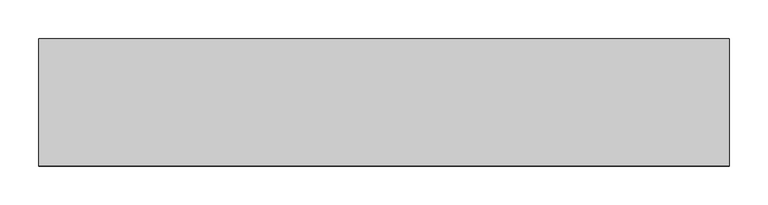
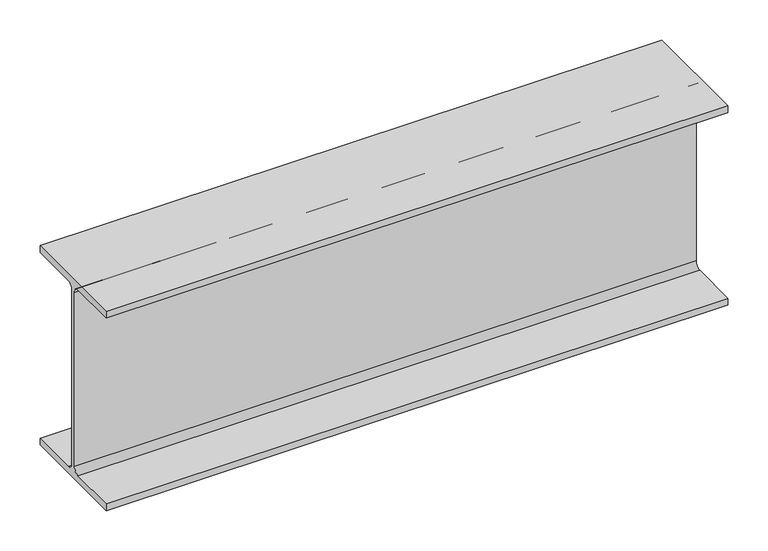
"""IFC4 building model written with IfcOpenShell, lengths in millimetres: beam geometry, Steel Beam_H-KSD3502 : H_SB_ASB_H-300x150x6.5x9."""

from ifc_helpers import new_model, si_unit, point, frame, frame_2d, origin, place, context, project, spatial, polyline, circle_curve, trimmed, segment, composite_curve, outline, extrude, source, transform, mapped, element, save


def beam_bd3552e1(model_context):
    return source(origin(), model_context, "Body", "SweptSolid", [
        extrude(outline(composite_curve([segment(polyline([(82.5, -141.5), (82.5, -151.7), (-82.5, -151.7), (-82.5, -141.5), (-11.9, -141.5)]), True, "CONTINUOUS"), segment(trimmed(circle_curve(frame_2d((-11.9, -132.6)), 8.9), [point((-11.9, -141.5))], [point((-3.0, -132.6))], True, "CARTESIAN"), True, "CONTINUOUS"), segment(polyline([(-3.0, -132.6), (-3.0, 132.6)]), True, "CONTINUOUS"), segment(trimmed(circle_curve(frame_2d((-11.9, 132.6)), 8.9), [point((-3.0, 132.6))], [point((-11.9, 141.5))], True, "CARTESIAN"), True, "CONTINUOUS"), segment(polyline([(-11.9, 141.5), (-82.5, 141.5), (-82.5, 151.7), (82.5, 151.7), (82.5, 141.5), (11.9, 141.5)]), True, "CONTINUOUS"), segment(trimmed(circle_curve(frame_2d((11.9, 132.6)), 8.9), [point((11.9, 141.5))], [point((3.0, 132.6))], True, "CARTESIAN"), True, "CONTINUOUS"), segment(polyline([(3.0, 132.6), (3.0, -132.6)]), True, "CONTINUOUS"), segment(trimmed(circle_curve(frame_2d((11.9, -132.6)), 8.9), [point((3.0, -132.6))], [point((11.9, -141.5))], True, "CARTESIAN"), True, "CONTINUOUS"), segment(polyline([(11.9, -141.5), (82.5, -141.5)]), True, "CONTINUOUS")], self_intersect=False)), frame((-349.8, 0.0, 0.0), z_axis=(1.0, 0.0, 0.0), x_axis=(0.0, 1.0, 0.0)), (0.0, 0.0, 1.0), 894.8),
    ])


if __name__ == "__main__":
    model = new_model("IFC4")
    model_context = context("Model", 3, world=origin())
    ifc_project = project(units=[si_unit("LENGTHUNIT", "METRE", prefix="MILLI")], contexts=[model_context])
    site = spatial("IfcSite", under=ifc_project)
    building = spatial("IfcBuilding", under=site)
    placement = place(None, origin())
    beam_shape = beam_bd3552e1(model_context)
    element("IfcBeam", 1, ObjectType="Steel Beam_H-KSD3502 : H_SB_ASB_H-300x150x6.5x9", at=placement, inside=building, context=model_context, shape_type="MappedRepresentation", body=[
        mapped(beam_shape, transform((0.0, 0.0, 0.0), x_axis=(1.0, 0.0, 0.0), y_axis=(0.0, 1.0, 0.0), z_axis=(0.0, 0.0, 1.0))),
    ])
    save(model, "model.ifc")

# Revit data of these elements
# Type "Steel Beam_H-KSD3502 : H_SB_ASB_H-300x150x6.5x9"
#   Width = 15.0 cm
#   Web Thickness = 0.65 cm
#   Web Fillet = 1.3 cm
#   Warping Constant = 107174.0 cm⁶
#   Torsional Moment of Inertia = 9.9539 cm⁴
#   Torsional Modulus = 1.0 cm³
#   Section Area = 46.78 cm²
#   Plastic Modulus weak axis = 105.0 cm³
#   Plastic Modulus strong axis = 542.0 cm³
#   Perimeter = 1.17 m²/m
#   Nominal Weight = 36.70 kgf/m
#   Moment of Inertia weak axis = 508.00 cm⁴
#   Moment of Inertia strong axis = 7210.00 cm⁴
#   Height = 30.0 cm
#   Flange Thickness = 0.9 cm
#   Elastic Modulus weak axis = 67.7 cm³
#   Elastic Modulus strong axis = 481.0 cm³
#   Centroid Vertical = 15.0 cm
#   Centroid Horizontal = 7.5 cm
#   Length [instance default] = 1.5240 m
#   Structural Material [instance default] = Steel, 45-345
#   Assembly Code = ""
# Element 1 (IfcBeam, "Steel Beam_H-KSD3502 : H_SB_ASB_H-300x150x6.5x9")
#   Structural Material = none
# Materials
#   "Steel, 45-345": class "Metal", colour RGB 189 187 185, transparency 0, Description = "Steel 345 MPa", Cost = 0
